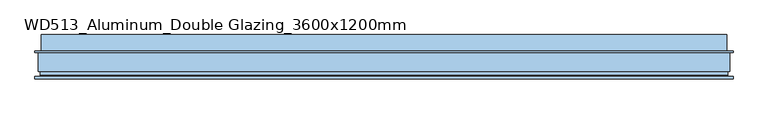
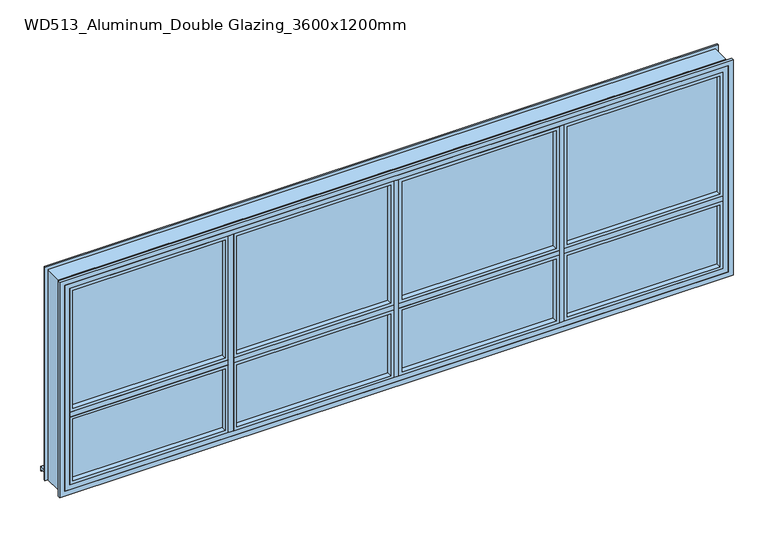
"""IFC4 building model written with IfcOpenShell, lengths in millimetres: window geometry, K-LINE ENSEMBLE COMPOSE NEUF KLT-8Z-4H2V : WD513_Aluminum_Double Glazing_3600x1200mm."""

from ifc_helpers import new_model, si_unit, frame, origin, place, context, project, spatial, polyline, outline, extrude, faceted_brep, source, transform, mapped, element, save


def wd513_aluminum_double_glazing_3600x1200mm_16f5b6b2(model_context):
    return source(origin(), model_context, "Body", "SolidModel", [
        extrude(outline(polyline([(-18.0, -155.0), (-18.0, -179.0), (-882.0, -179.0), (-882.0, -155.0), (-18.0, -155.0)])), frame((0.0, 0.0, 850.5), z_axis=(0.0, 0.0, 1.0), x_axis=(1.0, 0.0, 0.0)), (0.0, 0.0, 1.0), 381.5),
        extrude(outline(polyline([(1236.0, -14.0), (1236.0, -886.0), (846.5, -886.0), (846.5, -14.0), (1236.0, -14.0)]), holes=[polyline([(863.5, -31.0), (863.5, -869.0), (1219.0, -869.0), (1219.0, -31.0), (863.5, -31.0)])]), frame((0.0, -207.5, 0.0), z_axis=(0.0, 1.0, 0.0), x_axis=(0.0, 0.0, 1.0)), (0.0, 0.0, 1.0), 28.5),
        extrude(outline(polyline([(-18.0, -155.0), (-18.0, -179.0), (-882.0, -179.0), (-882.0, -155.0), (-18.0, -155.0)])), frame((0.0, 0.0, 1268.0), z_axis=(0.0, 0.0, 1.0), x_axis=(1.0, 0.0, 0.0)), (0.0, 0.0, 1.0), 705.0),
        extrude(outline(polyline([(1977.0, -14.0), (1977.0, -886.0), (1264.0, -886.0), (1264.0, -14.0), (1977.0, -14.0)]), holes=[polyline([(1281.0, -31.0), (1281.0, -869.0), (1960.0, -869.0), (1960.0, -31.0), (1281.0, -31.0)])]), frame((0.0, -207.5, 0.0), z_axis=(0.0, 1.0, 0.0), x_axis=(0.0, 0.0, 1.0)), (0.0, 0.0, 1.0), 28.5),
        extrude(outline(polyline([(-188.500001, 1241.0), (-188.500001, 1259.0), (-155.0, 1259.0), (-155.0, 1284.0), (-147.5, 1284.0), (-147.5, 1216.0), (-155.000001, 1216.0), (-155.000001, 1241.0), (-188.500001, 1241.0)])), frame((-866.0, 0.0, 0.0), z_axis=(1.0, 0.0, 0.0), x_axis=(0.0, 1.0, 0.0)), (0.0, 0.0, 1.0), 832.0),
        extrude(outline(polyline([(-14.0, -207.5), (-886.0, -207.5), (-886.0, -188.500001), (-14.0, -188.500001), (-14.0, -207.5)])), frame((0.0, 0.0, 1236.0), z_axis=(0.0, 0.0, 1.0), x_axis=(1.0, 0.0, 0.0)), (0.0, 0.0, 1.0), 28.0),
        extrude(outline(polyline([(-891.0, -155.0), (-891.0, -188.5), (-909.0, -188.5), (-909.0, -155.0), (-934.0, -155.0), (-934.0, -147.5), (-866.0, -147.5), (-866.0, -155.0), (-891.0, -155.0)])), frame((0.0, 0.0, 866.5), z_axis=(0.0, 0.0, 1.0), x_axis=(1.0, 0.0, 0.0)), (0.0, 0.0, 1.0), 1090.5),
        extrude(outline(polyline([(-914.0, -207.5), (-914.0, -188.5), (-886.0, -188.5), (-886.0, -207.5), (-914.0, -207.5)])), frame((0.0, 0.0, 846.5), z_axis=(0.0, 0.0, 1.0), x_axis=(1.0, 0.0, 0.0)), (0.0, 0.0, 1.0), 1130.5),
        extrude(outline(polyline([(882.0, -155.0), (882.0, -179.0), (18.0, -179.0), (18.0, -155.0), (882.0, -155.0)])), frame((0.0, 0.0, 850.5), z_axis=(0.0, 0.0, 1.0), x_axis=(1.0, 0.0, 0.0)), (0.0, 0.0, 1.0), 381.5),
        extrude(outline(polyline([(1236.0, 886.0), (1236.0, 14.0), (846.5, 14.0), (846.5, 886.0), (1236.0, 886.0)]), holes=[polyline([(863.5, 869.0), (863.5, 31.0), (1219.0, 31.0), (1219.0, 869.0), (863.5, 869.0)])]), frame((0.0, -207.5, 0.0), z_axis=(0.0, 1.0, 0.0), x_axis=(0.0, 0.0, 1.0)), (0.0, 0.0, 1.0), 28.5),
        extrude(outline(polyline([(882.0, -155.0), (882.0, -179.0), (18.0, -179.0), (18.0, -155.0), (882.0, -155.0)])), frame((0.0, 0.0, 1268.0), z_axis=(0.0, 0.0, 1.0), x_axis=(1.0, 0.0, 0.0)), (0.0, 0.0, 1.0), 705.0),
        extrude(outline(polyline([(1977.0, 886.0), (1977.0, 14.0), (1264.0, 14.0), (1264.0, 886.0), (1977.0, 886.0)]), holes=[polyline([(1281.0, 869.0), (1281.0, 31.0), (1960.0, 31.0), (1960.0, 869.0), (1281.0, 869.0)])]), frame((0.0, -207.5, 0.0), z_axis=(0.0, 1.0, 0.0), x_axis=(0.0, 0.0, 1.0)), (0.0, 0.0, 1.0), 28.5),
        extrude(outline(polyline([(-188.500001, 1241.0), (-188.500001, 1259.0), (-155.0, 1259.0), (-155.0, 1284.0), (-147.5, 1284.0), (-147.5, 1216.0), (-155.000001, 1216.0), (-155.000001, 1241.0), (-188.500001, 1241.0)])), frame((34.0, 0.0, 0.0), z_axis=(1.0, 0.0, 0.0), x_axis=(0.0, 1.0, 0.0)), (0.0, 0.0, 1.0), 832.0),
        extrude(outline(polyline([(886.0, -207.5), (14.0, -207.5), (14.0, -188.500001), (886.0, -188.500001), (886.0, -207.5)])), frame((0.0, 0.0, 1236.0), z_axis=(0.0, 0.0, 1.0), x_axis=(1.0, 0.0, 0.0)), (0.0, 0.0, 1.0), 28.0),
        extrude(outline(polyline([(9.0, -155.0), (9.0, -188.5), (-9.0, -188.5), (-9.0, -155.0), (-34.0, -155.0), (-34.0, -147.5), (34.0, -147.5), (34.0, -155.0), (9.0, -155.0)])), frame((0.0, 0.0, 866.5), z_axis=(0.0, 0.0, 1.0), x_axis=(1.0, 0.0, 0.0)), (0.0, 0.0, 1.0), 1090.5),
        extrude(outline(polyline([(-14.0, -207.5), (-14.0, -188.5), (14.0, -188.5), (14.0, -207.5), (-14.0, -207.5)])), frame((0.0, 0.0, 846.5), z_axis=(0.0, 0.0, 1.0), x_axis=(1.0, 0.0, 0.0)), (0.0, 0.0, 1.0), 1130.5),
        extrude(outline(polyline([(1773.0, -155.0), (1773.0, -179.0), (918.0, -179.0), (918.0, -155.0), (1773.0, -155.0)])), frame((0.0, 0.0, 850.5), z_axis=(0.0, 0.0, 1.0), x_axis=(1.0, 0.0, 0.0)), (0.0, 0.0, 1.0), 381.5),
        extrude(outline(polyline([(1236.0, 1777.0), (1236.0, 914.0), (846.5, 914.0), (846.5, 1777.0), (1236.0, 1777.0)]), holes=[polyline([(863.5, 1760.0), (863.5, 931.0), (1219.0, 931.0), (1219.0, 1760.0), (863.5, 1760.0)])]), frame((0.0, -207.5, 0.0), z_axis=(0.0, 1.0, 0.0), x_axis=(0.0, 0.0, 1.0)), (0.0, 0.0, 1.0), 28.5),
        extrude(outline(polyline([(-918.0, -155.0), (-918.0, -179.0), (-1773.0, -179.0), (-1773.0, -155.0), (-918.0, -155.0)])), frame((0.0, 0.0, 850.5), z_axis=(0.0, 0.0, 1.0), x_axis=(1.0, 0.0, 0.0)), (0.0, 0.0, 1.0), 381.5),
        extrude(outline(polyline([(1236.0, -914.0), (1236.0, -1777.0), (846.5, -1777.0), (846.5, -914.0), (1236.0, -914.0)]), holes=[polyline([(863.5, -931.0), (863.5, -1760.0), (1219.0, -1760.0), (1219.0, -931.0), (863.5, -931.0)])]), frame((0.0, -207.5, 0.0), z_axis=(0.0, 1.0, 0.0), x_axis=(0.0, 0.0, 1.0)), (0.0, 0.0, 1.0), 28.5),
        extrude(outline(polyline([(-188.500001, 1241.0), (-188.500001, 1259.0), (-155.0, 1259.0), (-155.0, 1284.0), (-147.5, 1284.0), (-147.5, 1216.0), (-155.000001, 1216.0), (-155.000001, 1241.0), (-188.500001, 1241.0)])), frame((-1757.0, 0.0, 0.0), z_axis=(1.0, 0.0, 0.0), x_axis=(0.0, 1.0, 0.0)), (0.0, 0.0, 1.0), 823.0),
        extrude(outline(polyline([(-914.0, -207.5), (-1777.0, -207.5), (-1777.0, -188.500001), (-914.0, -188.500001), (-914.0, -207.5)])), frame((0.0, 0.0, 1236.0), z_axis=(0.0, 0.0, 1.0), x_axis=(1.0, 0.0, 0.0)), (0.0, 0.0, 1.0), 28.0),
        extrude(outline(polyline([(-188.500001, 1241.0), (-188.500001, 1259.0), (-155.0, 1259.0), (-155.0, 1284.0), (-147.5, 1284.0), (-147.5, 1216.0), (-155.000001, 1216.0), (-155.000001, 1241.0), (-188.500001, 1241.0)])), frame((934.0, 0.0, 0.0), z_axis=(1.0, 0.0, 0.0), x_axis=(0.0, 1.0, 0.0)), (0.0, 0.0, 1.0), 823.0),
        extrude(outline(polyline([(1777.0, -207.5), (914.0, -207.5), (914.0, -188.500001), (1777.0, -188.500001), (1777.0, -207.5)])), frame((0.0, 0.0, 1236.0), z_axis=(0.0, 0.0, 1.0), x_axis=(1.0, 0.0, 0.0)), (0.0, 0.0, 1.0), 28.0),
        extrude(outline(polyline([(1773.0, -155.0), (1773.0, -179.0), (918.0, -179.0), (918.0, -155.0), (1773.0, -155.0)])), frame((0.0, 0.0, 1268.0), z_axis=(0.0, 0.0, 1.0), x_axis=(1.0, 0.0, 0.0)), (0.0, 0.0, 1.0), 705.0),
        extrude(outline(polyline([(1977.0, 1777.0), (1977.0, 914.0), (1264.0, 914.0), (1264.0, 1777.0), (1977.0, 1777.0)]), holes=[polyline([(1281.0, 1760.0), (1281.0, 931.0), (1960.0, 931.0), (1960.0, 1760.0), (1281.0, 1760.0)])]), frame((0.0, -207.5, 0.0), z_axis=(0.0, 1.0, 0.0), x_axis=(0.0, 0.0, 1.0)), (0.0, 0.0, 1.0), 28.5),
        extrude(outline(polyline([(-918.0, -155.0), (-918.0, -179.0), (-1773.0, -179.0), (-1773.0, -155.0), (-918.0, -155.0)])), frame((0.0, 0.0, 1268.0), z_axis=(0.0, 0.0, 1.0), x_axis=(1.0, 0.0, 0.0)), (0.0, 0.0, 1.0), 705.0),
        extrude(outline(polyline([(1977.0, -914.0), (1977.0, -1777.0), (1264.0, -1777.0), (1264.0, -914.0), (1977.0, -914.0)]), holes=[polyline([(1281.0, -931.0), (1281.0, -1760.0), (1960.0, -1760.0), (1960.0, -931.0), (1281.0, -931.0)])]), frame((0.0, -207.5, 0.0), z_axis=(0.0, 1.0, 0.0), x_axis=(0.0, 0.0, 1.0)), (0.0, 0.0, 1.0), 28.5),
        extrude(outline(polyline([(909.0, -155.0), (909.0, -188.5), (891.0, -188.5), (891.0, -155.0), (866.0, -155.0), (866.0, -147.5), (934.0, -147.5), (934.0, -155.0), (909.0, -155.0)])), frame((0.0, 0.0, 866.5), z_axis=(0.0, 0.0, 1.0), x_axis=(1.0, 0.0, 0.0)), (0.0, 0.0, 1.0), 1090.5),
        extrude(outline(polyline([(886.0, -207.5), (886.0, -188.5), (914.0, -188.5), (914.0, -207.5), (886.0, -207.5)])), frame((0.0, 0.0, 846.5), z_axis=(0.0, 0.0, 1.0), x_axis=(1.0, 0.0, 0.0)), (0.0, 0.0, 1.0), 1130.5),
        extrude(outline(polyline([(2032.0, 1832.0), (2032.0, -1832.0), (791.5, -1832.0), (791.5, 1832.0), (2032.0, 1832.0)]), holes=[polyline([(818.4999998, 1805.0000002), (818.4999998, -1805.0000002), (2005.0000002, -1805.0000002), (2005.0000002, 1805.0000002), (818.4999998, 1805.0000002)])]), frame((0.0, -207.5, 0.0), z_axis=(0.0, 1.0, 0.0), x_axis=(0.0, 0.0, 1.0)), (0.0, 0.0, 1.0), 12.5),
        extrude(outline(polyline([(2005.0000002, 1805.0000002), (2005.0000002, -1805.0000002), (818.4999998, -1805.0000002), (818.4999998, 1805.0000002), (2005.0000002, 1805.0000002)]), holes=[polyline([(846.5, 1777.0), (846.5, -1777.0), (1977.0, -1777.0), (1977.0, 1777.0), (846.5, 1777.0)])]), frame((0.0, -207.5, 0.0), z_axis=(0.0, 1.0, 0.0), x_axis=(0.0, 0.0, 1.0)), (0.0, 0.0, 1.0), 19.0),
        faceted_brep([(1756.999999, -154.9965859, 1956.999999), (1756.999999, -147.4965859, 1956.999999), (1756.999999, -147.4965859, 866.500001), (1756.999999, -154.9965859, 866.500001), (1805.0000002, -147.4965859, 818.4999998), (-1805.0000002, -147.4965859, 818.4999998), (-1805.0000002, -147.4965859, 2005.0000002), (1805.0000002, -147.4965859, 2005.0000002), (-1756.999999, -147.4965859, 1956.999999), (-1756.999999, -147.4965859, 866.500001), (-1756.999999, -154.9965859, 866.500001), (1782.0, -154.9965859, 1982.0), (-1782.0, -154.9965859, 1982.0), (-1782.0, -154.9965859, 841.5), (1782.0, -154.9965859, 841.5), (-1756.999999, -154.9965859, 1956.999999), (1782.0, -188.5, 1982.0), (1782.0, -188.5, 841.5), (-1782.0, -188.5, 841.5), (1805.0000002, -188.5, 2005.0000002), (-1805.0000002, -188.5, 2005.0000002), (-1805.0000002, -188.5, 818.4999998), (1805.0000002, -188.5, 818.4999998), (-1782.0, -188.5, 1982.0)], [[[0, 1, 2, 3]], [[4, 5, 6, 7], [1, 8, 9, 2]], [[3, 2, 9, 10]], [[11, 12, 13, 14], [3, 10, 15, 0]], [[16, 11, 14, 17]], [[17, 14, 13, 18]], [[19, 20, 21, 22], [17, 18, 23, 16]], [[7, 19, 22, 4]], [[4, 22, 21, 5]], [[10, 9, 8, 15]], [[18, 13, 12, 23]], [[5, 21, 20, 6]], [[15, 8, 1, 0]], [[23, 12, 11, 16]], [[6, 20, 19, 7]]]),
        faceted_brep([(-1815.0, -68.0, 805.0), (-1832.0, -68.0, 805.0), (-1832.0, -60.0, 805.0), (-1800.0, -60.0, 805.0), (-1800.0, -147.4965859, 805.0), (-1805.0, -147.4965859, 805.0), (-1805.0, -166.4965859, 805.0), (-1815.0, -166.4965859, 805.0), (-1815.0, -68.0, 2015.0), (1815.0, -68.0, 2015.0), (1815.0, -68.0, 805.0), (1832.0, -68.0, 805.0), (1832.0, -68.0, 2032.0), (-1832.0, -68.0, 2032.0), (-1832.0, -60.0, 2032.0), (1832.0, -60.0, 2032.0), (1832.0, -60.0, 805.0), (1800.0, -60.0, 805.0), (1800.0, -60.0, 2000.0), (-1800.0, -60.0, 2000.0), (-1800.0, -147.4965859, 2000.0), (1800.0, -147.4965859, 2000.0), (1800.0, -147.4965859, 805.0), (1805.0, -147.4965859, 805.0), (1805.0, -147.4965859, 2005.0), (-1805.0, -147.4965859, 2005.0), (-1805.0, -166.4965859, 2005.0), (1805.0, -166.4965859, 2005.0), (1805.0, -166.4965859, 805.0), (1815.0, -166.4965859, 805.0), (1815.0, -166.4965859, 2015.0), (-1815.0, -166.4965859, 2015.0)], [[[0, 1, 2, 3, 4, 5, 6, 7]], [[1, 0, 8, 9, 10, 11, 12, 13]], [[2, 1, 13, 14]], [[3, 2, 14, 15, 16, 17, 18, 19]], [[5, 4, 20, 21, 22, 23, 24, 25]], [[6, 5, 25, 26]], [[7, 6, 26, 27, 28, 29, 30, 31]], [[0, 7, 31, 8]], [[15, 12, 11, 16]], [[10, 29, 28, 23, 22, 17, 16, 11]], [[27, 24, 23, 28]], [[9, 30, 29, 10]], [[14, 13, 12, 15]], [[26, 25, 24, 27]], [[8, 31, 30, 9]], [[4, 3, 19, 20]], [[21, 18, 17, 22]], [[20, 19, 18, 21]]]),
        extrude(outline(polyline([(-147.4965859, 825.311129), (25.8038196, 819.2593455), (25.8038196, 794.3604516), (21.4038196, 794.3604516), (21.4038196, 805.0000004), (-161.2965876, 805.0000004), (-161.2965876, 818.5), (-147.4965859, 818.5), (-147.4965859, 825.311129)])), frame((-1800.0, 0.0, 0.0), z_axis=(1.0, 0.0, 0.0), x_axis=(0.0, 1.0, 0.0)), (0.0, 0.0, 1.0), 3600.0),
    ])


if __name__ == "__main__":
    model = new_model("IFC4")
    model_context = context("Model", 3, world=origin())
    ifc_project = project(units=[si_unit("LENGTHUNIT", "METRE", prefix="MILLI")], contexts=[model_context])
    site = spatial("IfcSite", under=ifc_project)
    building = spatial("IfcBuilding", under=site)
    placement = place(None, origin())
    wd513_aluminum_double_glazing_3600x1200mm_shape = wd513_aluminum_double_glazing_3600x1200mm_16f5b6b2(model_context)
    element("IfcWindow", 1, ObjectType="K-LINE ENSEMBLE COMPOSE NEUF KLT-8Z-4H2V : WD513_Aluminum_Double Glazing_3600x1200mm", at=placement, inside=building, context=model_context, shape_type="MappedRepresentation", body=[
        mapped(wd513_aluminum_double_glazing_3600x1200mm_shape, transform((0.0, 0.0, 0.0), x_axis=(1.0, 0.0, 0.0), y_axis=(0.0, 1.0, 0.0), z_axis=(0.0, 0.0, 1.0))),
    ])
    save(model, "model.ifc")

# Revit data of these elements
# Type "K-LINE ENSEMBLE COMPOSE NEUF KLT-8Z-4H2V : WD513_Aluminum_Double Glazing_3600x1200mm"
#   Type Mark = "AW"
#   Vitrage secondaire = ""
#   Vitrage principal = ""
#   URL = "https://pro.k-line.fr/bandes-ensembles-composes-kl-t.aspx"
#   Type de pose = "ITI"
#   Transmission lumineuse TLw = "67%"
#   SAV = "https://sav.k-line.fr/"
#   Product data url = "https://www.bimobject.com/k-line/product/klt-8zec2h4v"
#   Outil de thermo-luminosité = "http://www.pro.k-line.fr/calculateur-presentation.aspx"
#   Occultation = "Non"
#   Numéro de série = "K.........."
#   Keynote = "08520"
#   Neuf / Réno / Multi support = "Neuf"
#   Mortaise et grille d'entrée d'air = ""
#   Model = "KL-T Châssis Ensemble composé 8 Zones"
#   Matériaux = "Aluminium et verre"
#   Information renfort d'inertie = "Les renforts intérieurs ne sont compatible avec des ouvrants que sur des profils de 200mm de largeur"
#   Garanties = "https://pro.k-line.fr/pdf/attestations/Garanties_Legales_KLINE.pdf"
#   Famille de produit = "KL-City"
#   Manufacturer = "K.LINE"
#   Entretien = "https://pro.k-line.fr/pdf/ficheproduit/laq_fiche_entretien.pdf"
#   Entreprise de pose = ""
#   Doublages disponibles = "80,100,110,120,130,140,160,180 et 200 mm"
#   Description = "Fenêtre Alu"
#   Analytic Construction = "<Aucun>"
#   Composition analytique de base = "Châssis 1250x1480 - Vitrage 4/WE Argon 16/TBE 4 - Finition Black"
#   Classement AEV = "A*4 E*7B V*A3"
#   Classe COV = "A+"
#   Avis technique = "https://pro.k-line.fr/attestations-avis-technique.aspx"
#   Affaiblissement acoustique R(A,tr) = "30dB"
#   Val décal appui = 100 mm
#   Transmission thermique Uw = 1.4000 W/(m²·K)
#   Surface = 4.32 m²
#   Profondeur symbole d'ouverture = 150 mm
#   Position doublage = 0 mm
#   Lg traverse 4 = 909 mm
#   Lg traverse 3 = 918 mm
#   Lg traverse 2 = 918 mm
#   Lg traverse 1 = 909 mm
#   Largeur zone 4 = 900 mm
#   Largeur zone 3 = 900 mm
#   Largeur zone 2 = 900 mm
#   Largeur zone 1 = 900 mm
#   Largeur ouvrant 4 = 839 mm
#   Largeur ouvrant 3 = 848 mm
#   Largeur ouvrant 2 = 848 mm
#   Largeur ouvrant 1 = 839 mm
#   Rough Width [instance default] = 3600 mm
#   Largeur Traverse intermédiaire : 68,85,100,150,175 et 200 = 68 mm
#   Largeur Montant intermédiaire : 68,85,100,150,175 et 200 = 68 mm
#   Hauteur zone 5 = 750 mm
#   Hauteur zone 1 = 450 mm
#   Hauteur ouvrant 4/5/6 = 689 mm
#   Hauteur ouvrant 1/2/3 = 365.5 mm
#   Hauteur de poignée = 318 mm
#   Rough Height [instance default] = 1200 mm
#   Height = 1200 mm
#   Hauteur de l'appui par défaut = 800 mm
#   H profil = 1090.5 mm
#   Width = 3600 mm
#   Facteur solaire ScW (Hiver) = 0.53
#   Décalage appui = 180 mm
#   Décal appui = 40 mm
#   Doublage + ratrapage = 140 mm
#   Doublage = 140 mm
#   Centre zone 5/6/7/8 = 344.5 mm
#   Centre zone 1/2/3/4 = 182.75 mm
#   Centre Ouvrant 4/8 = 419.5 mm
#   Centre Ouvrant 3/7 = 450 mm
#   Centre Ouvrant 2/6 = 450 mm
#   Centre Ouvrant 1/5 = 419.5 mm
#   Angle symbole d'ouverture = 15.00°
#   Symbole d'ouverture = yes
#   Renfort saillant Intérieur = no
#   Renfort saillant Extérieur = no
#   Renfort Int saillant de 67.5 = no
#   Renfort Int saillant de 107.5 = yes
#   Renfort Ext saillant de 67.5 = no
#   Renfort Ext saillant de 107.5 = yes
#   Rattrapage doublage = no
#   Option appui sans aile intérieure = no
#   Finition Métal = yes
#   Finition Black = no
#   Rattrapage avec aile = no
#   Appui Non-Déporté = no
#   Appui Déporté = yes
#   Vitrage = Verre
#   Type d'ouvrant zone 8 = element 2302654
#   Type d'ouvrant zone 7 = element 2302654
#   Type d'ouvrant zone 6 = element 2302654
#   Type d'ouvrant zone 5 = element 2302654
#   Type d'ouvrant zone 4 = element 2302654
#   Type d'ouvrant zone 3 = element 2302654
#   Type d'ouvrant zone 2 = element 2302654
#   Type d'ouvrant zone 1 = element 2302654
#   Couleur panneau opaque Int = K.Line Intemporel Blanc satiné (9016 S) - KQ
#   Couleur panneau opaque Ext = K.Line Tendance Grège (9007 T) - RQ
#   Couleur châssis Int = K.Line Intemporel Blanc satiné (9016 S) - KQ
#   Couleur châssis Ext = K.Line Tendance Grège (9007 T) - RQ
#   Couleur Accessoire Int = K.Line Accessoire Blanc - KQ
#   Wall Closure = (empty or 0)
# Element 1 (IfcWindow, "K-LINE ENSEMBLE COMPOSE NEUF KLT-8Z-4H2V : WD513_Aluminum_Double Glazing_3600x1200mm")
#   Materials on its faces: "K.Line Intemporel Blanc satiné (9016 S) - KQ", "K.Line Tendance Grège (9007 T) - RQ", "Verre"
# Materials
#   "Verre": class "Verre", colour RGB 92 99 177, transparency 0.7, Description = "AL. WINDOW(TYP.)", Cost = 0
#   "K.Line Intemporel Blanc satiné (9016 S) - KQ": class "Metal", colour RGB 247 246 246, transparency 0, Description = "Aluminum 6061", Cost = 0
#   "K.Line Tendance Grège (9007 T) - RQ": class "Metal", colour RGB 135 133 129, transparency 0, Description = "Aluminum 6061", Cost = 0
#   "K.Line Accessoire Blanc - KQ": class "Metal", colour RGB 247 246 246, transparency 0, Description = "Aluminum 6061", Cost = 0
